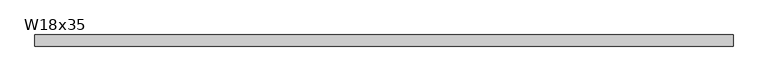
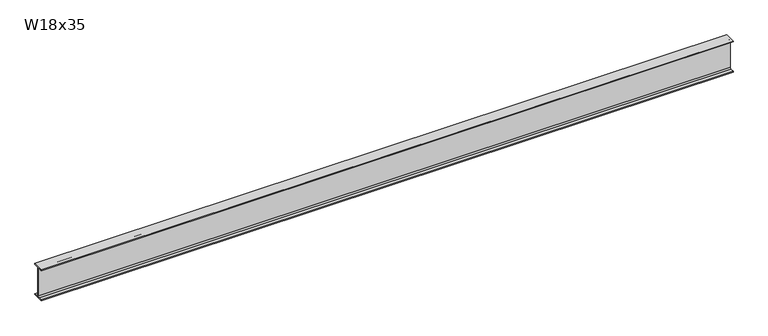
"""IFC4 building model written with IfcOpenShell, lengths in millimetres: beam geometry, RME W-Wide Flange : W18x35."""

from ifc_helpers import new_model, si_unit, point, frame, frame_2d, origin, place, context, project, spatial, polyline, circle_curve, trimmed, segment, composite_curve, outline, extrude, source, transform, mapped, element, save


def w18x35_ebe62907(model_context):
    return source(origin(), model_context, "Body", "SweptSolid", [
        extrude(outline(composite_curve([segment(polyline([(76.2, -213.995), (76.2, -224.79), (-76.2, -224.79), (-76.2, -213.995), (-21.59, -213.995)]), True, "CONTINUOUS"), segment(trimmed(circle_curve(frame_2d((-21.59, -196.215)), 17.78), [point((-21.59, -213.995))], [point((-3.81, -196.215))], True, "CARTESIAN"), True, "CONTINUOUS"), segment(polyline([(-3.81, -196.215), (-3.81, 196.215)]), True, "CONTINUOUS"), segment(trimmed(circle_curve(frame_2d((-21.59, 196.215)), 17.78), [point((-3.81, 196.215))], [point((-21.59, 213.995))], True, "CARTESIAN"), True, "CONTINUOUS"), segment(polyline([(-21.59, 213.995), (-76.2, 213.995), (-76.2, 224.79), (76.2, 224.79), (76.2, 213.995), (21.59, 213.995)]), True, "CONTINUOUS"), segment(trimmed(circle_curve(frame_2d((21.59, 196.215)), 17.78), [point((21.59, 213.995))], [point((3.81, 196.215))], True, "CARTESIAN"), True, "CONTINUOUS"), segment(polyline([(3.81, 196.215), (3.81, -196.215)]), True, "CONTINUOUS"), segment(trimmed(circle_curve(frame_2d((21.59, -196.215)), 17.78), [point((3.81, -196.215))], [point((21.59, -213.995))], True, "CARTESIAN"), True, "CONTINUOUS"), segment(polyline([(21.59, -213.995), (76.2, -213.995)]), True, "CONTINUOUS")], self_intersect=False)), frame((-4763.389, 0.0, 0.0), z_axis=(1.0, 0.0, 0.0), x_axis=(0.0, 1.0, 0.0)), (0.0, 0.0, 1.0), 9526.778),
    ])


if __name__ == "__main__":
    model = new_model("IFC4")
    model_context = context("Model", 3, world=origin())
    ifc_project = project(units=[si_unit("LENGTHUNIT", "METRE", prefix="MILLI")], contexts=[model_context])
    site = spatial("IfcSite", under=ifc_project)
    building = spatial("IfcBuilding", under=site)
    placement = place(None, origin())
    w18x35_shape = w18x35_ebe62907(model_context)
    element("IfcBeam", 1, ObjectType="RME W-Wide Flange : W18x35", at=placement, inside=building, context=model_context, shape_type="MappedRepresentation", body=[
        mapped(w18x35_shape, transform((0.0, 0.0, 0.0), x_axis=(1.0, 0.0, 0.0), y_axis=(0.0, 1.0, 0.0), z_axis=(0.0, 0.0, 1.0))),
    ])
    save(model, "model.ifc")

# Revit data of these elements
# Type "RME W-Wide Flange : W18x35"
#   WELD P [instance default] = ""
#   WELD LE [instance default] = ""
#   WELD D [instance default] = ""
#   TOP SECTION SIZE [instance default] = ""
#   TOP SECTION LENGTH [instance default] = ""
#   REMARKS [instance default] = ""
#   REINF TYPE [instance default] = ""
#   Nominal Size = "W24"
#   End Bearing Capacity [instance default] = ""
#   BOT SECTION SIZE [instance default] = ""
#   BOT SECTION LENGTH [instance default] = ""
#   Assembly Code = "B10"
#   W = 35
#   Start Extension Calculation [instance default] = 10' - 0"
#   Start Extension [instance default] = -0' - 0 1/2"
#   End Extension Calculation [instance default] = 10' - 0"
#   End Extension [instance default] = -0' - 0 1/2"
#   Length [instance default] = 5' - 0"
#   bf = 0' - 6"
#   d = 1' - 5.7"
#   k = 0' - 1 1/8"
#   k2 = 0' - 0.7"
#   tf = 0' - 0.425"
#   tw = 0' - 0.3"
#   A = 0.0715278 SF
#   Structural Material [instance default] = Metal - Steel - ASTM A992
# Element 1 (IfcBeam, "RME W-Wide Flange : W18x35")
#   Length = 32' - 0"
#   Materials on its faces: "Metal - Steel - ASTM A992"
# Materials
#   "Metal - Steel - ASTM A992": class "Metal", colour RGB 255 128 0, transparency 0
